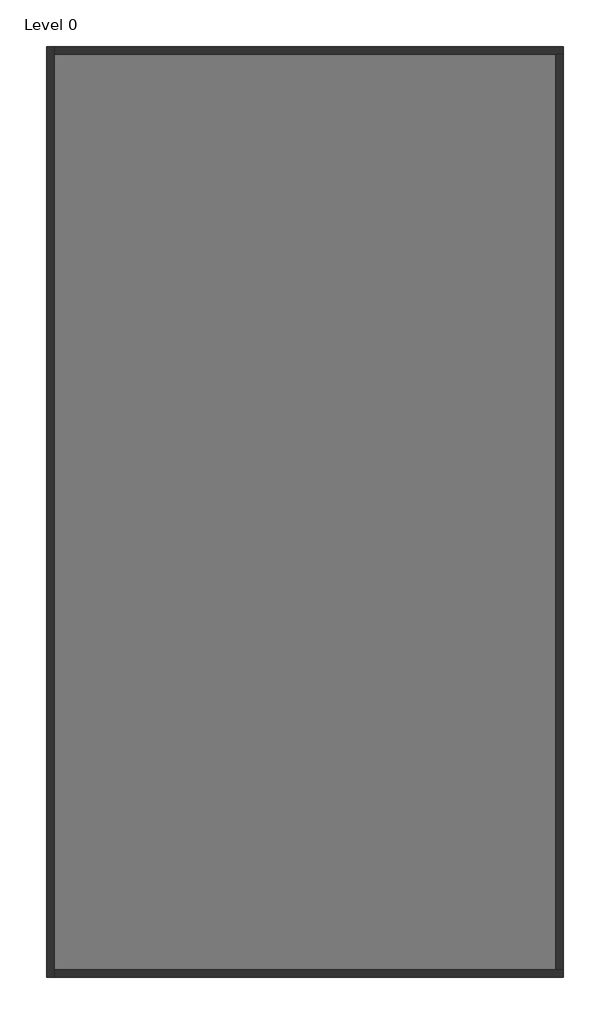
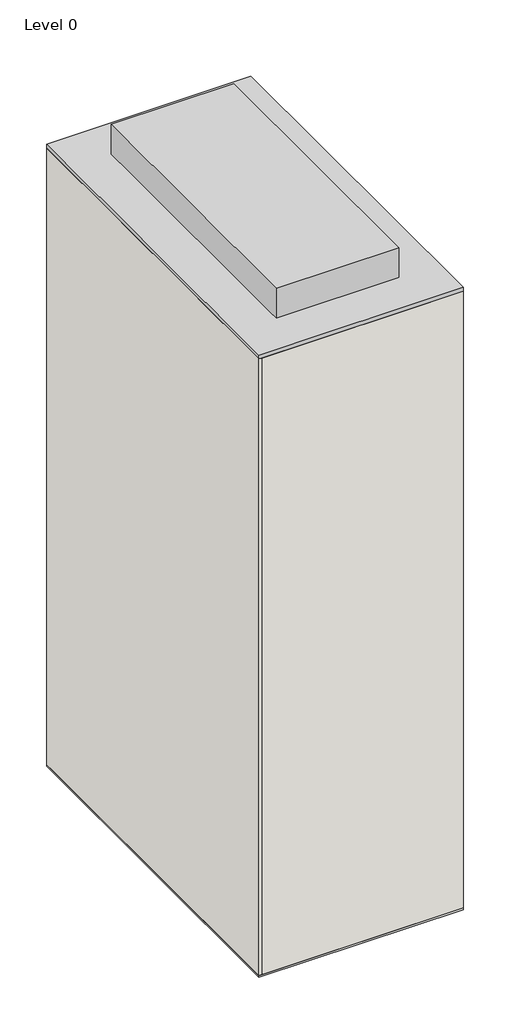
# One storey: 4 walls, 1 proxy, 1 slab.
"""IFC4 building model written with IfcOpenShell, lengths in millimetres."""

from ifc_helpers import new_model, si_unit, frame, origin, origin_with_axes, place, context, project, spatial, polyline, outline, extrude, faceted_brep, element, save

model = new_model("IFC4")

# Units and contexts
model_context = context("Model", 3, world=origin())
ifc_project = project(units=[si_unit("LENGTHUNIT", "METRE", prefix="MILLI")], contexts=[model_context])

# Site, building, storey
site = spatial("IfcSite", under=ifc_project)
building = spatial("IfcBuilding", under=site)
storey = spatial("IfcBuildingStorey", under=building, Name="Level 0", Elevation=100.0)

# Proxy
placement = place(None, origin())
element("IfcBuildingElementProxy", 1, Name="LowUrbanDensityBuilding : LowUrbanDensityBuilding", ObjectType="LowUrbanDensityBuilding : LowUrbanDensityBuilding", at=placement, inside=storey, context=model_context, shape_type="SweptSolid", body=[
    extrude(outline(polyline([(7325.2659446, 3676.2074539), (7325.2659446, -14323.7925461), (-2674.7340554, -14323.7925461), (-2674.7340554, 3676.2074539), (7325.2659446, 3676.2074539)])), origin_with_axes(), (0.0, 0.0, 1.0), 32200.0),
    extrude(outline(polyline([(5325.2659446, 1676.2074539), (5325.2659446, -12323.7925461), (-674.7340554, -12323.7925461), (-674.7340554, 1676.2074539), (5325.2659446, 1676.2074539)])), frame((0.0, 0.0, 32000.0), z_axis=(0.0, 0.0, 1.0), x_axis=(1.0, 0.0, 0.0)), (0.0, 0.0, 1.0), 1749.8),
])

# Slab
element("IfcSlab", 2, ObjectType="Floor-Concrete_100Con", at=placement, inside=storey, context=model_context, shape_type="SweptSolid", body=[
    extrude(outline(polyline([(7325.2659446, 3676.2074539), (7325.2659446, -14323.7925461), (-2674.7340554, -14323.7925461), (-2674.7340554, 3676.2074539), (7325.2659446, 3676.2074539)])), origin_with_axes(), (0.0, 0.0, 1.0), 100.0),
])

# Walls
element("IfcWall", 3, ObjectType="Wall-Ext_25Rdr-100Blk-19P", at=placement, inside=storey, context=model_context, shape_type="Brep", body=[
    faceted_brep([(-2674.7340554, 3676.2074539, 100.0), (-2674.7340554, -14323.7925461, 100.0), (-2674.7340554, -14323.7925461, 32000.0), (-2674.7340554, 3676.2074539, 32000.0), (-2530.4340554, 3676.2074539, 100.0), (-2530.4340554, 3676.2074539, 32000.0), (-2530.4340554, 3531.9074539, 32000.0), (-2530.4340554, -14179.4925461, 32000.0), (-2530.4340554, -14323.7925461, 32000.0), (-2530.4340554, -14323.7925461, 100.0), (-2530.4340554, -14179.4925461, 100.0), (-2530.4340554, 3531.9074539, 100.0)], [[[0, 1, 2, 3]], [[4, 5, 6, 7, 8, 9, 10, 11]], [[1, 0, 4, 11, 10, 9]], [[3, 2, 8, 7, 6, 5]], [[2, 1, 9, 8]], [[0, 3, 5, 4]]]),
])
element("IfcWall", 4, ObjectType="Wall-Ext_25Rdr-100Blk-19P", at=placement, inside=storey, context=model_context, shape_type="Brep", body=[
    faceted_brep([(-2530.4340554, -14323.7925461, 100.0), (7325.2659446, -14323.7925461, 100.0), (7325.2659446, -14323.7925461, 32000.0), (-2530.4340554, -14323.7925461, 32000.0), (-2530.4340554, -14179.4925461, 100.0), (-2530.4340554, -14179.4925461, 32000.0), (7180.9659446, -14179.4925461, 32000.0), (7325.2659446, -14179.4925461, 32000.0), (7325.2659446, -14179.4925461, 100.0), (7180.9659446, -14179.4925461, 100.0)], [[[0, 1, 2, 3]], [[4, 5, 6, 7, 8, 9]], [[1, 0, 4, 9, 8]], [[3, 2, 7, 6, 5]], [[0, 3, 5, 4]], [[2, 1, 8, 7]]]),
])
element("IfcWall", 5, ObjectType="Wall-Ext_25Rdr-100Blk-19P", at=placement, inside=storey, context=model_context, shape_type="Brep", body=[
    faceted_brep([(7325.2659446, 3676.2074539, 100.0), (-2530.4340554, 3676.2074539, 100.0), (-2530.4340554, 3676.2074539, 32000.0), (7325.2659446, 3676.2074539, 32000.0), (7325.2659446, 3531.9074539, 100.0), (7325.2659446, 3531.9074539, 32000.0), (7180.9659446, 3531.9074539, 32000.0), (-2530.4340554, 3531.9074539, 32000.0), (-2530.4340554, 3531.9074539, 100.0), (7180.9659446, 3531.9074539, 100.0)], [[[0, 1, 2, 3]], [[4, 5, 6, 7, 8, 9]], [[1, 0, 4, 9, 8]], [[3, 2, 7, 6, 5]], [[2, 1, 8, 7]], [[0, 3, 5, 4]]]),
])
element("IfcWall", 6, ObjectType="Wall-Ext_25Rdr-100Blk-19P", at=placement, inside=storey, context=model_context, shape_type="SweptSolid", body=[
    extrude(outline(polyline([(7325.2659446, 3531.9074539), (7325.2659446, -14179.4925461), (7180.9659446, -14179.4925461), (7180.9659446, 3531.9074539), (7325.2659446, 3531.9074539)])), frame((0.0, 0.0, 100.0), z_axis=(0.0, 0.0, 1.0), x_axis=(1.0, 0.0, 0.0)), (0.0, 0.0, 1.0), 31900.0),
])

save(model, "model.ifc")

# Revit data of these elements
# Project information
#   Project Issue Date = "Issue Date"
#   Project Status = "Project Status"
#   Client Name = "Owner"
#   Project Address = "Enter address here"
#   Project Name = "Project Name"
#   Project Number = "Project Number"
# Type "Floor-Concrete_100Con"
#   Keynote = "E60/130"
#   Function = 0
#   Layers, outside or top first: 100 mm "Concrete" (function 1)
# Type "Wall-Ext_25Rdr-100Blk-19P"
#   Keynote = "F10"
#   Layers, outside or top first: 25.3 mm "Render, Beige, Smooth" (function 5); 100 mm "Concrete Masonry Units _Low Density" (function 1); 19 mm "Plaster" (function 5)
# Element 1 (IfcBuildingElementProxy, "LowUrbanDensityBuilding : LowUrbanDensityBuilding")
#   Phase Created = New Construction
#   Materials on its faces: "Default Form"
# Element 2 (IfcSlab, "Floor-Concrete_100Con")
#   Height Offset From Level = 0 mm
#   Phase Created = New Construction
#   Materials on its faces: "Concrete"
# Element 3 (IfcWall, "Wall-Ext_25Rdr-100Blk-19P")
#   Top Offset = 0 mm
#   Base Offset = 0 mm
#   wall height = 31900 mm
#   Phase Created = New Construction
#   Base Constraint = Level 0
#   Top Constraint = Level 8
#   Materials on its faces: "Render, Beige, Smooth", "Default Wall", "Plaster"
# Elements 4, 5, 6 (IfcWall, "Wall-Ext_25Rdr-100Blk-19P")
#   Top Offset = 0 mm
#   Base Offset = 0 mm
#   wall height = 31900 mm
#   Phase Created = New Construction
#   Base Constraint = Level 0
#   Top Constraint = Level 8
#   Materials on its faces: "Default Wall", "Render, Beige, Smooth", "Plaster"
# Materials
#   "Concrete": class "Concrete", colour RGB 120 120 120, transparency 0, Description = "Portland Cement Concrete", Cost = 0
#   "Render, Beige, Smooth": class "Generic", colour RGB 213 198 180, transparency 0, Description = "physical material", Cost = 0
#   "Concrete Masonry Units _Low Density": class "Masonry", colour RGB 181 181 181, transparency 0, Description = "Concrete masonry units", Cost = 0
#   "Plaster": class "Generic", colour RGB 249 249 249, transparency 0, Description = "Plaster", Cost = 0
#   "Default Form": class "Generic", colour RGB 185 189 196, transparency 0.5, Cost = 0
#   "Default Wall": class "Miscellaneous", colour RGB 128 128 128, transparency 0, Comments = "Rendering appearance not upgraded Rendering appearance not upgraded ", Cost = 0
